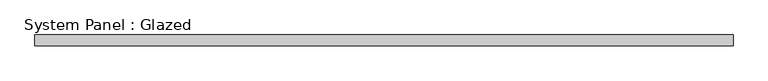
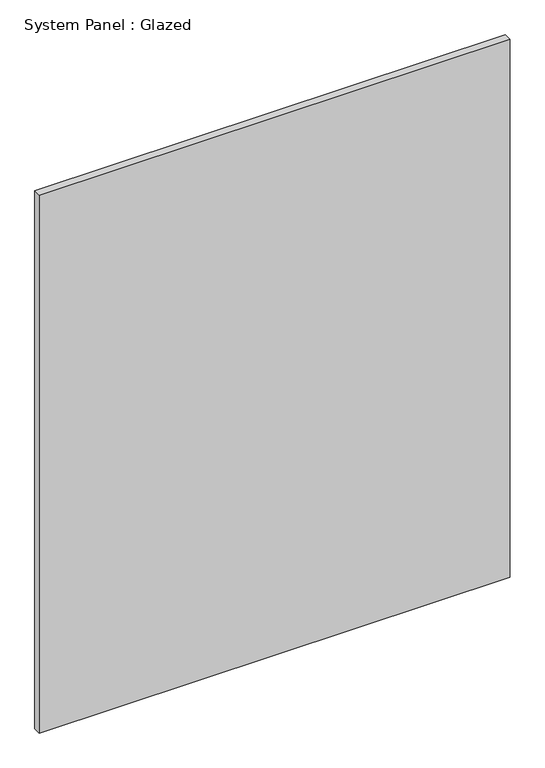
"""IFC4 building model written with IfcOpenShell, lengths in millimetres: plate geometry, System Panel : Glazed."""

from ifc_helpers import new_model, si_unit, origin, origin_with_axes, place, context, project, spatial, polyline, outline, extrude, source, transform, mapped, element, save


def system_panel_glazed_e9a9ab38(model_context):
    return source(origin(), model_context, "Body", "SweptSolid", [
        extrude(outline(polyline([(807.5, 24.5), (-807.5, 24.5), (-807.5, 49.5), (807.5, 49.5), (807.5, 24.5)])), origin_with_axes(), (0.0, 0.0, 1.0), 1950.0),
    ])


if __name__ == "__main__":
    model = new_model("IFC4")
    model_context = context("Model", 3, world=origin())
    ifc_project = project(units=[si_unit("LENGTHUNIT", "METRE", prefix="MILLI")], contexts=[model_context])
    site = spatial("IfcSite", under=ifc_project)
    building = spatial("IfcBuilding", under=site)
    placement = place(None, origin())
    system_panel_glazed_shape = system_panel_glazed_e9a9ab38(model_context)
    element("IfcPlate", 1, ObjectType="System Panel : Glazed", at=placement, inside=building, context=model_context, shape_type="MappedRepresentation", body=[
        mapped(system_panel_glazed_shape, transform((0.0, 0.0, 0.0), x_axis=(1.0, 0.0, 0.0), y_axis=(0.0, 1.0, 0.0), z_axis=(0.0, 0.0, 1.0))),
    ])
    save(model, "model.ifc")

# Revit data of these elements
# Element 1 (IfcPlate, "System Panel : Glazed")
#   Materials on its faces: "Glass"
# Materials
#   "Glass": class "Glass", colour RGB 0 128 192, transparency 0.9
